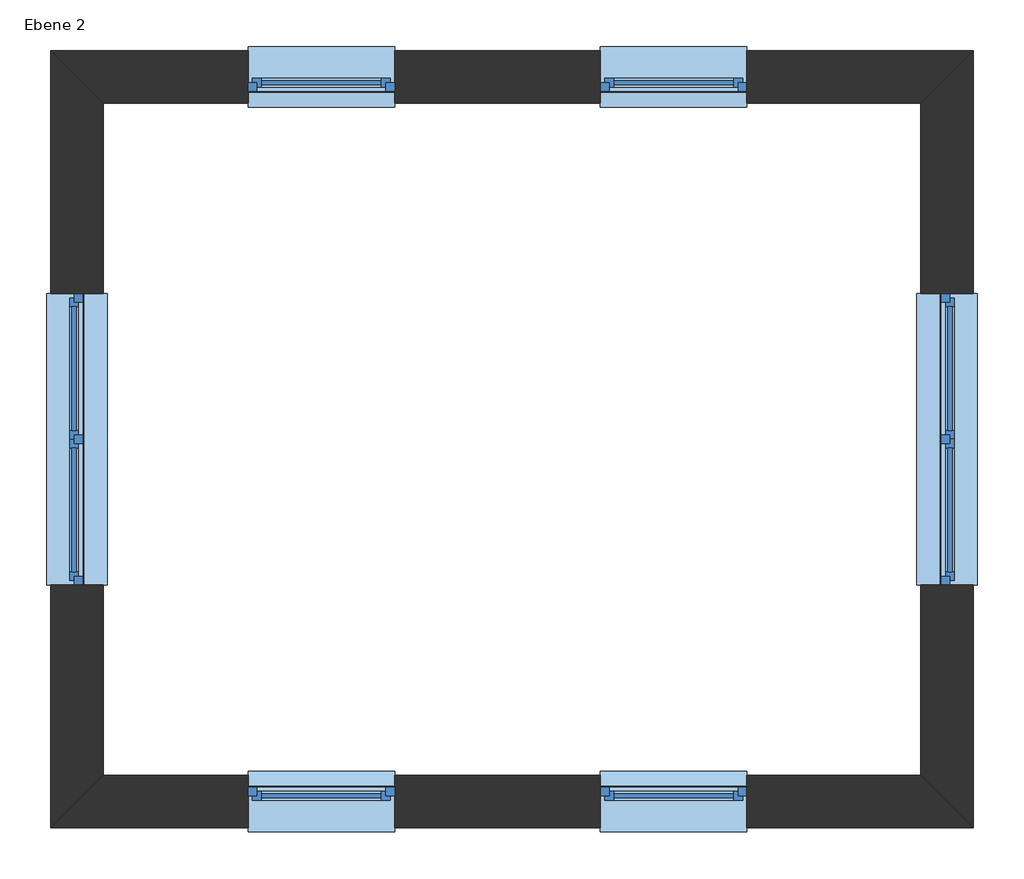
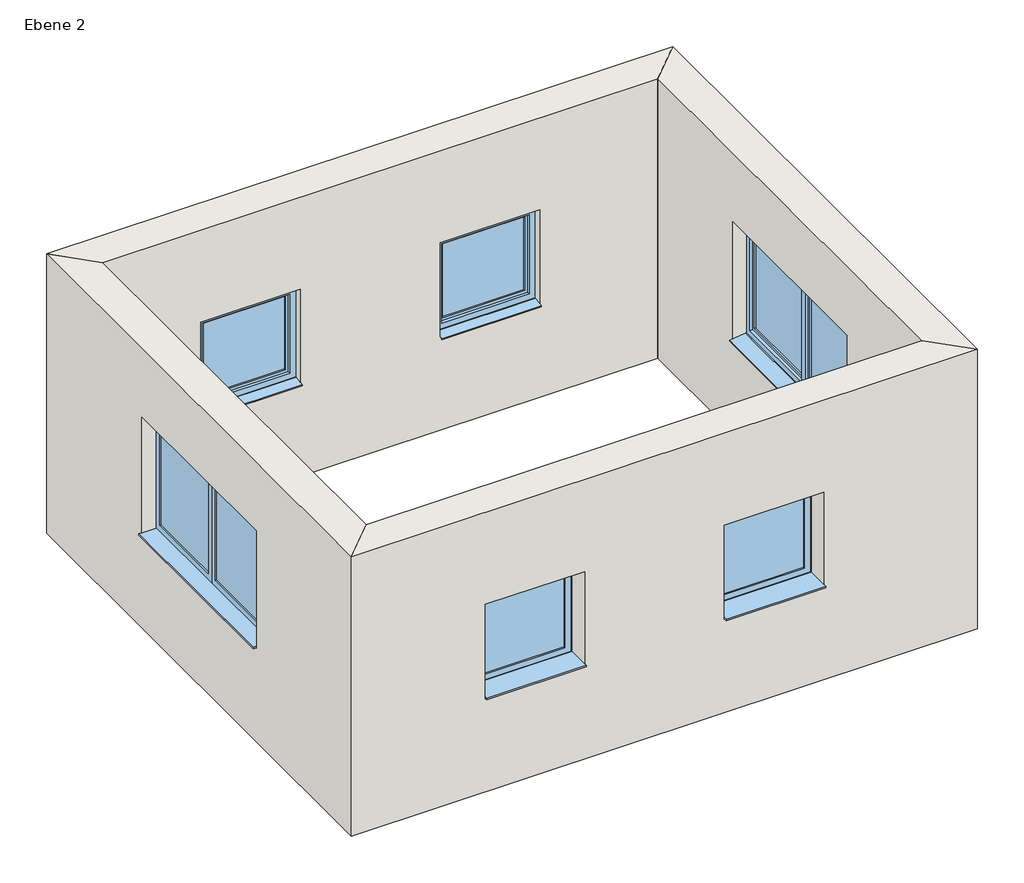
# One storey: 6 windows, 4 walls.
"""IFC4 building model written with IfcOpenShell, lengths in millimetres."""

import ifcopenshell
import ifcopenshell.guid

model = None  # the IFC model being written
_history = None  # IfcOwnerHistory: only IFC2X3 demands one
_inside = {}  # id of a spatial element -> (the spatial element, [elements in it])
_under = {}  # id of a project, library or spatial element -> (it, [spatial elements below it])
_declared = {}  # id of a project -> (the project, [libraries it declares])
_typed = {}  # id of a type object -> (the type object, [elements of that type])
_made_of = {}  # id of a material, layer set ... -> (it, [elements and type objects made of it])


def new_model(schema):
    """Start an empty IFC model of exactly this schema.

    Asked for "IFC4X3", IfcOpenShell would pick the latest addendum, in which some entities
    have other attributes; the version numbers below select the first issue.
    IFC2X3 requires an IfcOwnerHistory on every rooted entity: one is made here for all.
    """
    global model, _history
    if schema == "IFC4X3":
        model = ifcopenshell.file(schema_version=(4, 3, 0, 0))
    else:
        model = ifcopenshell.file(schema=schema)
    _inside.clear()
    _under.clear()
    _declared.clear()
    _typed.clear()
    _made_of.clear()
    _history = None
    if model.schema == "IFC2X3":
        org = make("IfcOrganization", Name="unknown")
        user = make(
            "IfcPersonAndOrganization",
            ThePerson=make("IfcPerson", FamilyName="unknown"),
            TheOrganization=org,
        )
        app = make(
            "IfcApplication",
            ApplicationDeveloper=org,
            Version="unknown",
            ApplicationFullName="unknown",
            ApplicationIdentifier="unknown",
        )
        _history = make(
            "IfcOwnerHistory",
            OwningUser=user,
            OwningApplication=app,
            ChangeAction="ADDED",
            CreationDate=0,
        )
    return model


def make(cls, **values):
    """One entity of the class cls with the attributes given. An attribute that is None is left unset."""
    return model.create_entity(
        cls, **{name: value for name, value in values.items() if value is not None}
    )


def rooted(cls, **values):
    """An entity with a GlobalId (a new one), such as an element, a storey or a relation."""
    return make(cls, GlobalId=ifcopenshell.guid.new(), OwnerHistory=_history, **values)


def si_unit(unit_type, name, prefix=None):
    """IfcSIUnit, for example si_unit("LENGTHUNIT", "METRE", prefix="MILLI")."""
    return make("IfcSIUnit", UnitType=unit_type, Prefix=prefix, Name=name)


def assignment(units):
    """IfcUnitAssignment: the units of a project."""
    return None if units is None else make("IfcUnitAssignment", Units=units)


def point(xyz):
    """IfcCartesianPoint."""
    return None if xyz is None else make("IfcCartesianPoint", Coordinates=xyz)


def direction(xyz):
    """IfcDirection."""
    return None if xyz is None else make("IfcDirection", DirectionRatios=xyz)


def frame(location, z_axis=None, x_axis=None):
    """IfcAxis2Placement3D, a coordinate frame: its origin and axes. An axis left out is left unset."""
    return make(
        "IfcAxis2Placement3D",
        Location=point(location),
        Axis=direction(z_axis),
        RefDirection=direction(x_axis),
    )


def origin():
    """The frame at (0, 0, 0) with its axes left unset."""
    return frame((0.0, 0.0, 0.0))


def place(relative_to, where):
    """IfcLocalPlacement: puts the frame where relative to a parent placement (None: the world)."""
    return make(
        "IfcLocalPlacement", PlacementRelTo=relative_to, RelativePlacement=where
    )


def context(
    kind, dimensions, precision=None, world=None, true_north=None, identifier=None
):
    """IfcGeometricRepresentationContext, for example the 3D "Model" context."""
    return make(
        "IfcGeometricRepresentationContext",
        ContextIdentifier=identifier,
        ContextType=kind,
        CoordinateSpaceDimension=dimensions,
        Precision=precision,
        WorldCoordinateSystem=world,
        TrueNorth=true_north,
    )


def project(units=None, contexts=None):
    """IfcProject with its units and contexts."""
    return rooted(
        "IfcProject",
        Name="project",
        RepresentationContexts=contexts,
        UnitsInContext=assignment(units),
    )


def spatial(cls, under=None, at=None, **own):
    """A site, building, storey or space (cls), placed at a placement, below another one or the project."""
    s = rooted(cls, ObjectPlacement=at, **own)
    if under is not None:
        _under.setdefault(under.id(), (under, []))[1].append(s)
    return s


def polyline(points):
    """IfcPolyline through the points."""
    return make("IfcPolyline", Points=[point(p) for p in points])


def outline(outer, holes=None, kind="AREA"):
    """IfcArbitraryClosedProfileDef: a profile drawn as a closed curve; with holes, ...WithVoids."""
    if holes is None:
        return make("IfcArbitraryClosedProfileDef", ProfileType=kind, OuterCurve=outer)
    return make(
        "IfcArbitraryProfileDefWithVoids",
        ProfileType=kind,
        OuterCurve=outer,
        InnerCurves=holes,
    )


def extrude(swept, where, along, depth):
    """IfcExtrudedAreaSolid: the profile swept, set in the frame where, extruded along a direction by depth."""
    return make(
        "IfcExtrudedAreaSolid",
        SweptArea=swept,
        Position=where,
        ExtrudedDirection=direction(along),
        Depth=depth,
    )


def faces_of(points, faces, orient=None, outer=None):
    """IfcFace entities. A face is a list of loops; a loop is a list of indices into points, from 0.

    orient and outer hold one flag for each loop. By default every Orientation is true, the
    first loop of a face is its IfcFaceOuterBound and the others are IfcFaceBound.
    """
    made = []
    for i, loops in enumerate(faces):
        bounds = []
        for j, loop in enumerate(loops):
            is_outer = j == 0 if outer is None else outer[i][j]
            bounds.append(
                make(
                    "IfcFaceOuterBound" if is_outer else "IfcFaceBound",
                    Bound=make("IfcPolyLoop", Polygon=[points[k] for k in loop]),
                    Orientation=True if orient is None else orient[i][j],
                )
            )
        made.append(make("IfcFace", Bounds=bounds))
    return made


def faceted_brep(points, faces, orient=None, outer=None, voids=None):
    """IfcFacetedBrep: a solid bounded by flat faces; with voids (closed shells), ...WithVoids."""
    shared = [point(p) for p in points]
    hull = make("IfcClosedShell", CfsFaces=faces_of(shared, faces, orient, outer))
    if voids is None:
        return make("IfcFacetedBrep", Outer=hull)
    return make(
        "IfcFacetedBrepWithVoids",
        Outer=hull,
        Voids=[
            make(cls, CfsFaces=faces_of(shared, fs, o, b)) for cls, fs, o, b in voids
        ],
    )


def shape(context_of_items, identifier, shape_type, items):
    """IfcShapeRepresentation: the items that make up one representation, for example the "Body"."""
    return make(
        "IfcShapeRepresentation",
        ContextOfItems=context_of_items,
        RepresentationIdentifier=identifier,
        RepresentationType=shape_type,
        Items=items,
    )


def source(mapping_origin, context_of_items, identifier, shape_type, items):
    """IfcRepresentationMap: a shape defined once, which mapped items show again and again."""
    return make(
        "IfcRepresentationMap",
        MappingOrigin=mapping_origin,
        MappedRepresentation=shape(context_of_items, identifier, shape_type, items),
    )


def transform(
    local_origin,
    x_axis=None,
    y_axis=None,
    z_axis=None,
    scale=None,
    scale2=None,
    scale3=None,
    uniform=True,
):
    """IfcCartesianTransformationOperator3D, or its non-uniform kind. x_axis, y_axis, z_axis: its Axis1, 2, 3."""
    if uniform:
        return make(
            "IfcCartesianTransformationOperator3D",
            Axis1=direction(x_axis),
            Axis2=direction(y_axis),
            LocalOrigin=point(local_origin),
            Scale=scale,
            Axis3=direction(z_axis),
        )
    return make(
        "IfcCartesianTransformationOperator3DnonUniform",
        Axis1=direction(x_axis),
        Axis2=direction(y_axis),
        LocalOrigin=point(local_origin),
        Scale=scale,
        Axis3=direction(z_axis),
        Scale2=scale2,
        Scale3=scale3,
    )


def mapped(mapping_source, mapping_target):
    """IfcMappedItem: shows the shape of a source again, moved by a transform."""
    return make(
        "IfcMappedItem", MappingSource=mapping_source, MappingTarget=mapping_target
    )


def made_of(thing, what):
    """Note that an element or type object is made of a material, layer set ...; save() writes the relation."""
    if what is not None:
        _made_of.setdefault(what.id(), (what, []))[1].append(thing)
    return thing


def element(
    cls,
    number,
    at=None,
    inside=None,
    cuts=None,
    type_object=None,
    material=None,
    context=None,
    identifier="Body",
    shape_type=None,
    held_by="IfcProductDefinitionShape",
    body=None,
    shapes=None,
    **own,
):
    """One element of the class cls, such as IfcWall. Its Tag is "e" and its number.

    at: its placement. inside: the storey or other place that contains it. cuts: it is an
    opening in that element (IfcRelVoidsElement). A single representation is given by context,
    identifier, shape_type and body (its items); several are given by shapes. held_by: the class
    of the entity that holds the representations. save() writes the other relations.
    """
    e = rooted(cls, Tag="e%d" % number, ObjectPlacement=at, **own)
    if body is not None:
        shapes = [shape(context, identifier, shape_type, body)]
    if shapes is not None:
        e.Representation = make(held_by, Representations=shapes)
    if inside is not None:
        _inside.setdefault(inside.id(), (inside, []))[1].append(e)
    if cuts is not None:
        rooted(
            "IfcRelVoidsElement", RelatingBuildingElement=cuts, RelatedOpeningElement=e
        )
    if type_object is not None:
        _typed.setdefault(type_object.id(), (type_object, []))[1].append(e)
    return made_of(e, material)


def aggregate(whole, parts):
    """IfcRelAggregates: a whole, such as a stair, and the parts it consists of."""
    return rooted("IfcRelAggregates", RelatingObject=whole, RelatedObjects=parts)


def save(model, path):
    """Write the relations noted so far, then the file.

    IfcRelAggregates (storeys below a building ...), IfcRelContainedInSpatialStructure (elements
    in a storey), IfcRelDefinesByType, IfcRelAssociatesMaterial and IfcRelDeclares: one each for
    every whole, place, type object, material and project.
    """
    for whole, parts in _under.values():
        aggregate(whole, parts)
    for where, things in _inside.values():
        rooted(
            "IfcRelContainedInSpatialStructure",
            RelatedElements=things,
            RelatingStructure=where,
        )
    for kind, things in _typed.values():
        rooted("IfcRelDefinesByType", RelatedObjects=things, RelatingType=kind)
    for what, things in _made_of.values():
        rooted("IfcRelAssociatesMaterial", RelatedObjects=things, RelatingMaterial=what)
    for by, libraries in _declared.values():
        rooted("IfcRelDeclares", RelatingContext=by, RelatedDefinitions=libraries)
    model.write(path)


def fenster_1_flg_variabel_fenster_1_flg_variabel_3_8a378bad(model_context):
    return source(origin(), model_context, "Body", "SolidModel", [
        extrude(outline(polyline([(2010.0, 505.0), (2010.0, -505.0), (1000.0, -505.0), (1000.0, 505.0), (2010.0, 505.0)]), holes=[polyline([(1930.0, 445.0), (1080.0, 445.0), (1080.0, -445.0), (1930.0, -445.0), (1930.0, 445.0)])]), frame((0.0, 40.0, 0.0), z_axis=(0.0, 1.0, 0.0), x_axis=(0.0, 0.0, 1.0)), (0.0, 0.0, 1.0), 60.0),
        faceted_brep([(475.0, 40.0, 1960.0), (475.0, 10.0, 1960.0), (475.0, 10.0, 1050.0), (475.0, 40.0, 1050.0), (-475.0, 10.0, 1960.0), (-475.0, 10.0, 1050.0), (415.0, 10.0, 1110.0), (-415.0, 10.0, 1110.0), (-415.0, 10.0, 1900.0), (415.0, 10.0, 1900.0), (-475.0, 40.0, 1050.0), (-475.0, 40.0, 1960.0), (445.0, 40.0, 1930.0), (-445.0, 40.0, 1930.0), (-445.0, 40.0, 1080.0), (445.0, 40.0, 1080.0), (445.0, 70.0, 1930.0), (445.0, 70.0, 1080.0), (-445.0, 70.0, 1080.0), (-445.0, 70.0, 1930.0), (415.0, 70.0, 1900.0), (-415.0, 70.0, 1900.0), (-415.0, 70.0, 1110.0), (415.0, 70.0, 1110.0)], [[[0, 1, 2, 3]], [[1, 4, 5, 2], [6, 7, 8, 9]], [[3, 2, 5, 10]], [[3, 10, 11, 0], [12, 13, 14, 15]], [[16, 12, 15, 17]], [[17, 15, 14, 18]], [[17, 18, 19, 16], [20, 21, 22, 23]], [[9, 20, 23, 6]], [[6, 23, 22, 7]], [[10, 5, 4, 11]], [[18, 14, 13, 19]], [[7, 22, 21, 8]], [[11, 4, 1, 0]], [[19, 13, 12, 16]], [[8, 21, 20, 9]]]),
        extrude(outline(polyline([(-505.0, -210.0), (-505.0, 40.0), (505.0, 40.0), (505.0, -210.0), (-505.0, -210.0)])), frame((0.0, 0.0, 1005.0), z_axis=(0.0, 0.0, 1.0), x_axis=(1.0, 0.0, 0.0)), (0.0, 0.0, 1.0), 15.0),
        extrude(outline(polyline([(110.0221543, 1020.0), (210.0, 1000.0), (210.0, 990.0), (208.0, 990.0), (208.0, 998.3604634), (109.8240723, 1018.0), (100.0, 1018.0), (100.0, 1020.0), (110.0221543, 1020.0)])), frame((-505.0, 0.0, 0.0), z_axis=(1.0, 0.0, 0.0), x_axis=(0.0, 1.0, 0.0)), (0.0, 0.0, 1.0), 1010.0),
        extrude(outline(polyline([(415.0, 25.0), (-415.0, 25.0), (-415.0, 55.0), (415.0, 55.0), (415.0, 25.0)])), frame((0.0, 0.0, 1110.0), z_axis=(0.0, 0.0, 1.0), x_axis=(1.0, 0.0, 0.0)), (0.0, 0.0, 1.0), 790.0),
    ])


def fenster_2_flg_variabel_fenster_2_flg_variabel_3_03287464(model_context):
    return source(origin(), model_context, "Body", "SolidModel", [
        extrude(outline(polyline([(60.0, -5.0), (915.0, -5.0), (915.0, -35.0), (60.0, -35.0), (60.0, -5.0)])), frame((0.0, 0.0, 1110.0), z_axis=(0.0, 0.0, 1.0), x_axis=(1.0, 0.0, 0.0)), (0.0, 0.0, 1.0), 1040.0),
        extrude(outline(polyline([(-915.0, -5.0), (-60.0, -5.0), (-60.0, -35.0), (-915.0, -35.0), (-915.0, -5.0)])), frame((0.0, 0.0, 1110.0), z_axis=(0.0, 0.0, 1.0), x_axis=(1.0, 0.0, 0.0)), (0.0, 0.0, 1.0), 1040.0),
        extrude(outline(polyline([(-1005.0, -210.0), (-1005.0, -20.0), (1005.0, -20.0), (1005.0, -210.0), (-1005.0, -210.0)])), frame((0.0, 0.0, 1005.0), z_axis=(0.0, 0.0, 1.0), x_axis=(1.0, 0.0, 0.0)), (0.0, 0.0, 1.0), 15.0),
        extrude(outline(polyline([(50.0221543, 1020.0), (210.0, 1000.0), (210.0, 990.0), (208.0, 990.0), (208.0, 998.3604634), (49.8240723, 1018.0), (40.0, 1018.0), (40.0, 1020.0), (50.0221543, 1020.0)])), frame((-1005.0, 0.0, 0.0), z_axis=(1.0, 0.0, 0.0), x_axis=(0.0, 1.0, 0.0)), (0.0, 0.0, 1.0), 2010.0),
        extrude(outline(polyline([(30.0, -20.0), (-30.0, -20.0), (-30.0, 40.0), (30.0, 40.0), (30.0, -20.0)])), frame((0.0, 0.0, 1080.0), z_axis=(0.0, 0.0, 1.0), x_axis=(1.0, 0.0, 0.0)), (0.0, 0.0, 1.0), 1100.0),
        extrude(outline(polyline([(2260.0, -1005.0), (1000.0, -1005.0), (1000.0, 1005.0), (2260.0, 1005.0), (2260.0, -1005.0)]), holes=[polyline([(2180.0, -945.0), (2180.0, 945.0), (1080.0, 945.0), (1080.0, -945.0), (2180.0, -945.0)])]), frame((0.0, -20.0, 0.0), z_axis=(0.0, 1.0, 0.0), x_axis=(0.0, 0.0, 1.0)), (0.0, 0.0, 1.0), 60.0),
        faceted_brep([(-945.0, -20.0, 1080.0), (-945.0, 10.0, 1080.0), (-30.0, 10.0, 1080.0), (-30.0, -20.0, 1080.0), (-30.0, 10.0, 2180.0), (-30.0, -20.0, 2180.0), (-945.0, 10.0, 2180.0), (-60.0, 10.0, 2150.0), (-915.0, 10.0, 2150.0), (-915.0, 10.0, 1110.0), (-60.0, 10.0, 1110.0), (0.0, -20.0, 1050.0), (-975.0, -20.0, 1050.0), (-975.0, -20.0, 2210.0), (0.0, -20.0, 2210.0), (-945.0, -20.0, 2180.0), (-975.0, -50.0, 1050.0), (0.0, -50.0, 1050.0), (0.0, -50.0, 2210.0), (-975.0, -50.0, 2210.0), (-60.0, -50.0, 1110.0), (-915.0, -50.0, 1110.0), (-915.0, -50.0, 2150.0), (-60.0, -50.0, 2150.0)], [[[0, 1, 2, 3]], [[3, 2, 4, 5]], [[2, 1, 6, 4], [7, 8, 9, 10]], [[11, 12, 13, 14], [5, 15, 0, 3]], [[16, 12, 11, 17]], [[17, 11, 14, 18]], [[18, 19, 16, 17], [20, 21, 22, 23]], [[9, 21, 20, 10]], [[10, 20, 23, 7]], [[15, 6, 1, 0]], [[19, 13, 12, 16]], [[8, 22, 21, 9]], [[5, 4, 6, 15]], [[18, 14, 13, 19]], [[7, 23, 22, 8]]]),
        faceted_brep([(30.0, -20.0, 1080.0), (30.0, 10.0, 1080.0), (945.0, 10.0, 1080.0), (945.0, -20.0, 1080.0), (945.0, 10.0, 2180.0), (945.0, -20.0, 2180.0), (30.0, 10.0, 2180.0), (915.0, 10.0, 2150.0), (60.0, 10.0, 2150.0), (60.0, 10.0, 1110.0), (915.0, 10.0, 1110.0), (975.0, -20.0, 1050.0), (0.0, -20.0, 1050.0), (0.0, -20.0, 2210.0), (975.0, -20.0, 2210.0), (30.0, -20.0, 2180.0), (0.0, -50.0, 1050.0), (975.0, -50.0, 1050.0), (975.0, -50.0, 2210.0), (0.0, -50.0, 2210.0), (915.0, -50.0, 1110.0), (60.0, -50.0, 1110.0), (60.0, -50.0, 2150.0), (915.0, -50.0, 2150.0)], [[[0, 1, 2, 3]], [[3, 2, 4, 5]], [[2, 1, 6, 4], [7, 8, 9, 10]], [[11, 12, 13, 14], [5, 15, 0, 3]], [[16, 12, 11, 17]], [[17, 11, 14, 18]], [[18, 19, 16, 17], [20, 21, 22, 23]], [[9, 21, 20, 10]], [[10, 20, 23, 7]], [[15, 6, 1, 0]], [[19, 13, 12, 16]], [[8, 22, 21, 9]], [[5, 4, 6, 15]], [[18, 14, 13, 19]], [[7, 23, 22, 8]]]),
    ])


model = new_model("IFC4")

# Units and contexts
model_context = context("Model", 3, world=origin())
ifc_project = project(units=[si_unit("LENGTHUNIT", "METRE", prefix="MILLI")], contexts=[model_context])

# Site, building, storey
site = spatial("IfcSite", under=ifc_project)
building = spatial("IfcBuilding", under=site)
storey = spatial("IfcBuildingStorey", under=building, Name="Ebene 2", Elevation=6000.0)

# Walls
placement = place(None, origin())
element("IfcWall", 1, ObjectType="MW 24.0 WD 12.0", at=placement, inside=storey, context=model_context, shape_type="Brep", body=[
    faceted_brep([(-3766.4979049, 4044.3692517, 6000.0), (1873.5020951, 4044.3692517, 6000.0), (1873.5020951, 4044.3692517, 9000.0), (-3766.4979049, 4044.3692517, 9000.0), (673.5020951, 4044.3692517, 7000.0), (-336.4979049, 4044.3692517, 7000.0), (-336.4979049, 4044.3692517, 8010.0), (673.5020951, 4044.3692517, 8010.0), (-1756.4979049, 4044.3692517, 7000.0), (-2766.4979049, 4044.3692517, 7000.0), (-2766.4979049, 4044.3692517, 8010.0), (-1756.4979049, 4044.3692517, 8010.0), (-4126.4979049, 4404.3692517, 6000.0), (-4126.4979049, 4404.3692517, 9000.0), (2233.5020951, 4404.3692517, 9000.0), (2233.5020951, 4404.3692517, 6000.0), (673.5020951, 4404.3692517, 7000.0), (673.5020951, 4404.3692517, 8010.0), (-336.4979049, 4404.3692517, 8010.0), (-336.4979049, 4404.3692517, 7000.0), (-1756.4979049, 4404.3692517, 7000.0), (-1756.4979049, 4404.3692517, 8010.0), (-2766.4979049, 4404.3692517, 8010.0), (-2766.4979049, 4404.3692517, 7000.0)], [[[0, 1, 2, 3], [4, 5, 6, 7], [8, 9, 10, 11]], [[12, 13, 14, 15], [16, 17, 18, 19], [20, 21, 22, 23]], [[1, 0, 12, 15]], [[3, 2, 14, 13]], [[2, 1, 15, 14]], [[0, 3, 13, 12]], [[17, 16, 4, 7]], [[18, 17, 7, 6]], [[19, 18, 6, 5]], [[16, 19, 5, 4]], [[21, 20, 8, 11]], [[22, 21, 11, 10]], [[23, 22, 10, 9]], [[20, 23, 9, 8]]]),
])
element("IfcWall", 2, ObjectType="MW 24.0 WD 12.0", at=placement, inside=storey, context=model_context, shape_type="Brep", body=[
    faceted_brep([(1873.5020951, 4044.3692517, 6000.0), (1873.5020951, -595.6307483, 6000.0), (1873.5020951, -595.6307483, 9000.0), (1873.5020951, 4044.3692517, 9000.0), (1873.5020951, 719.3692517, 7000.0), (1873.5020951, 2729.3692517, 7000.0), (1873.5020951, 2729.3692517, 8260.0), (1873.5020951, 719.3692517, 8260.0), (2233.5020951, 4404.3692517, 6000.0), (2233.5020951, 4404.3692517, 9000.0), (2233.5020951, -955.6307483, 9000.0), (2233.5020951, -955.6307483, 6000.0), (2233.5020951, 719.3692517, 7000.0), (2233.5020951, 719.3692517, 8260.0), (2233.5020951, 2729.3692517, 8260.0), (2233.5020951, 2729.3692517, 7000.0)], [[[0, 1, 2, 3], [4, 5, 6, 7]], [[8, 9, 10, 11], [12, 13, 14, 15]], [[1, 0, 8, 11]], [[3, 2, 10, 9]], [[0, 3, 9, 8]], [[2, 1, 11, 10]], [[13, 12, 4, 7]], [[14, 13, 7, 6]], [[15, 14, 6, 5]], [[12, 15, 5, 4]]]),
])
element("IfcWall", 3, ObjectType="MW 24.0 WD 12.0", at=placement, inside=storey, context=model_context, shape_type="Brep", body=[
    faceted_brep([(1873.5020951, -595.6307483, 6000.0), (-3766.4979049, -595.6307483, 6000.0), (-3766.4979049, -595.6307483, 9000.0), (1873.5020951, -595.6307483, 9000.0), (-336.4979049, -595.6307483, 7000.0), (673.5020951, -595.6307483, 7000.0), (673.5020951, -595.6307483, 8010.0), (-336.4979049, -595.6307483, 8010.0), (-2766.4979049, -595.6307483, 7000.0), (-1756.4979049, -595.6307483, 7000.0), (-1756.4979049, -595.6307483, 8010.0), (-2766.4979049, -595.6307483, 8010.0), (2233.5020951, -955.6307483, 6000.0), (2233.5020951, -955.6307483, 9000.0), (-4126.4979049, -955.6307483, 9000.0), (-4126.4979049, -955.6307483, 6000.0), (-336.4979049, -955.6307483, 7000.0), (-336.4979049, -955.6307483, 8010.0), (673.5020951, -955.6307483, 8010.0), (673.5020951, -955.6307483, 7000.0), (-2766.4979049, -955.6307483, 7000.0), (-2766.4979049, -955.6307483, 8010.0), (-1756.4979049, -955.6307483, 8010.0), (-1756.4979049, -955.6307483, 7000.0)], [[[0, 1, 2, 3], [4, 5, 6, 7], [8, 9, 10, 11]], [[12, 13, 14, 15], [16, 17, 18, 19], [20, 21, 22, 23]], [[1, 0, 12, 15]], [[3, 2, 14, 13]], [[0, 3, 13, 12]], [[2, 1, 15, 14]], [[17, 16, 4, 7]], [[18, 17, 7, 6]], [[19, 18, 6, 5]], [[16, 19, 5, 4]], [[21, 20, 8, 11]], [[22, 21, 11, 10]], [[23, 22, 10, 9]], [[20, 23, 9, 8]]]),
])
element("IfcWall", 4, ObjectType="MW 24.0 WD 12.0", at=placement, inside=storey, context=model_context, shape_type="Brep", body=[
    faceted_brep([(-3766.4979049, -595.6307483, 6000.0), (-3766.4979049, 4044.3692517, 6000.0), (-3766.4979049, 4044.3692517, 9000.0), (-3766.4979049, -595.6307483, 9000.0), (-3766.4979049, 2729.3692517, 7000.0), (-3766.4979049, 719.3692517, 7000.0), (-3766.4979049, 719.3692517, 8260.0), (-3766.4979049, 2729.3692517, 8260.0), (-4126.4979049, -955.6307483, 6000.0), (-4126.4979049, -955.6307483, 9000.0), (-4126.4979049, 4404.3692517, 9000.0), (-4126.4979049, 4404.3692517, 6000.0), (-4126.4979049, 2729.3692517, 7000.0), (-4126.4979049, 2729.3692517, 8260.0), (-4126.4979049, 719.3692517, 8260.0), (-4126.4979049, 719.3692517, 7000.0)], [[[0, 1, 2, 3], [4, 5, 6, 7]], [[8, 9, 10, 11], [12, 13, 14, 15]], [[1, 0, 8, 11]], [[3, 2, 10, 9]], [[2, 1, 11, 10]], [[0, 3, 9, 8]], [[13, 12, 4, 7]], [[14, 13, 7, 6]], [[15, 14, 6, 5]], [[12, 15, 5, 4]]]),
])

# Windows
fenster_1_flg_variabel_fenster_1_flg_variabel_3_shape = fenster_1_flg_variabel_fenster_1_flg_variabel_3_8a378bad(model_context)
element("IfcWindow", 5, ObjectType="Fenster 1-flg - Variabel : Fenster 1-flg - Variabel 3", at=placement, inside=storey, context=model_context, shape_type="MappedRepresentation", body=[
    mapped(fenster_1_flg_variabel_fenster_1_flg_variabel_3_shape, transform((168.5020951, -775.6307483, 6000.0), x_axis=(1.0, 0.0, 0.0), y_axis=(0.0, 1.0, 0.0), z_axis=(0.0, 0.0, 1.0))),
])
element("IfcWindow", 6, ObjectType="Fenster 1-flg - Variabel : Fenster 1-flg - Variabel 3", at=placement, inside=storey, context=model_context, shape_type="MappedRepresentation", body=[
    mapped(fenster_1_flg_variabel_fenster_1_flg_variabel_3_shape, transform((-2261.4979049, -775.6307483, 6000.0), x_axis=(1.0, 0.0, 0.0), y_axis=(0.0, 1.0, 0.0), z_axis=(0.0, 0.0, 1.0))),
])
element("IfcWindow", 7, ObjectType="Fenster 1-flg - Variabel : Fenster 1-flg - Variabel 3", at=placement, inside=storey, context=model_context, shape_type="MappedRepresentation", body=[
    mapped(fenster_1_flg_variabel_fenster_1_flg_variabel_3_shape, transform((168.5020951, 4224.3692517, 6000.0), x_axis=(-1.0, 0.0, 0.0), y_axis=(0.0, -1.0, 0.0), z_axis=(0.0, 0.0, 1.0))),
])
element("IfcWindow", 8, ObjectType="Fenster 1-flg - Variabel : Fenster 1-flg - Variabel 3", at=placement, inside=storey, context=model_context, shape_type="MappedRepresentation", body=[
    mapped(fenster_1_flg_variabel_fenster_1_flg_variabel_3_shape, transform((-2261.4979049, 4224.3692517, 6000.0), x_axis=(-1.0, 0.0, 0.0), y_axis=(0.0, -1.0, 0.0), z_axis=(0.0, 0.0, 1.0))),
])
fenster_2_flg_variabel_fenster_2_flg_variabel_3_shape = fenster_2_flg_variabel_fenster_2_flg_variabel_3_03287464(model_context)
element("IfcWindow", 9, ObjectType="Fenster 2-flg - Variabel : Fenster 2-flg - Variabel 3", at=placement, inside=storey, context=model_context, shape_type="MappedRepresentation", body=[
    mapped(fenster_2_flg_variabel_fenster_2_flg_variabel_3_shape, transform((2053.5020951, 1724.3692517, 6000.0), x_axis=(0.0, 1.0, 0.0), y_axis=(-1.0, 0.0, 0.0), z_axis=(0.0, 0.0, 1.0))),
])
element("IfcWindow", 10, ObjectType="Fenster 2-flg - Variabel : Fenster 2-flg - Variabel 3", at=placement, inside=storey, context=model_context, shape_type="MappedRepresentation", body=[
    mapped(fenster_2_flg_variabel_fenster_2_flg_variabel_3_shape, transform((-3946.4979049, 1724.3692517, 6000.0), x_axis=(0.0, -1.0, 0.0), y_axis=(1.0, 0.0, 0.0), z_axis=(0.0, 0.0, 1.0))),
])

save(model, "model.ifc")

# Revit data of these elements
# Type "MW 24.0 WD 12.0"
#   Type Comments = "Mehrschaliges Mauerwerk"
#   Description = "Mauerwerk 24.0 cm, Wärmedämmung 12.0 cm"
#   Layers, outside or top first: 0.120 m "Wärmedämmung - hart" (function 3); 0.240 m "Mauerwerk - Ziegel, verputzt" (function 1)
# Type "Fenster 1-flg - Variabel : Fenster 1-flg - Variabel 3"
#   Type Mark = "52"
#   Operation = "SinglePanel"
#   Construction Type Id = "GSP4R"
#   Keynote = "16.05.01"
#   Analytic Construction = "1/8 Zoll Pilkington-Verglasung einfach"
#   Cost = 78.2
#   Visual Light Transmittance = 0.9
#   Höhe oberer  Rahmen = 0.080 m
#   Solar Heat Gain Coefficient = 0.86
#   Tiefe Flügel = 0.060 m
#   Rough Width [instance default] = 1.010 m
#   Rough Height [instance default] = 1.010 m
#   Rahmenhöhe unten = 0.080 m
#   Heat Transfer Coefficient (U) = 6.7069 W/(m²·K)
#   Rahmentiefe = 0.060 m
#   Rahmenbreite = 0.060 m
#   Height [instance default] = 1.010 m
#   Flügelbreite = 0.060 m
#   Einbautiefe (von außen) [instance default] = 0.080 m
#   Width [instance default] = 1.010 m
#   Define Thermal Properties by = 1
#   Öffnungsrichtung oben [instance default] = yes
#   Öffnungsrichtung in Draufsicht anzeigen [instance default] = no
#   Klappflügel [instance default] = no
#   Drehflügel 1 [instance default] = yes
#   Fensterflügel [instance default] = none
#   Innere Fensterbank [instance default] = none
#   Glas [instance default] = none
#   Bild [instance default] = none
#   Äußere Fensterbank [instance default] = none
#   Wall Closure = (empty or 0)
# Type "Fenster 2-flg - Variabel : Fenster 2-flg - Variabel 3"
#   Type Mark = "53"
#   Operation = "DoublePanelVertical"
#   Construction Type Id = "GSP4R"
#   Keynote = "16.05.01"
#   Analytic Construction = "1/8 Zoll Pilkington-Verglasung einfach"
#   Cost = 130.98
#   Visual Light Transmittance = 0.9
#   Solar Heat Gain Coefficient = 0.78
#   Rough Width [instance default] = 2.010 m
#   Rough Height [instance default] = 1.260 m
#   Heat Transfer Coefficient (U) = 3.6886 W/(m²·K)
#   Rahmentiefe = 0.060 m
#   Rahmenhöhe unten = 0.080 m
#   Höhe oberer  Rahmen = 0.080 m
#   Rahmenbreite = 0.060 m
#   Height [instance default] = 1.260 m
#   Tiefe Flügel = 0.060 m
#   Flügelbreite = 0.060 m
#   Einbautiefe (von außen) [instance default] = 0.140 m
#   Width [instance default] = 2.010 m
#   Define Thermal Properties by = 1
#   Öffnungsrichtung oben [instance default] = yes
#   Öffnungsrichtung in Draufsicht anzeigen [instance default] = no
#   Drehflügel 1 [instance default] = yes
#   Bild [instance default] = none
#   Glas [instance default] = none
#   Fensterflügel [instance default] = none
#   Äußere Fensterbank [instance default] = none
#   Innere Fensterbank [instance default] = none
#   Wall Closure = (empty or 0)
# Elements 1, 2, 3, 4 (IfcWall, "MW 24.0 WD 12.0")
#   Comments = ""
#   Top Offset = 0.000 m
#   Base Offset = 0.000 m
#   Unconnected Height = 3.000 m
#   wall height = 3.000 m
#   Phase Created = Phase 1
#   Base Constraint = Ebene 2
#   Materials on its faces: "Vorgabe - Wand", "Mauerwerk - Ziegel, verputzt", "Wärmedämmung - hart"
# Element 5 (IfcWindow, "Fenster 1-flg - Variabel : Fenster 1-flg - Variabel 3")
#   Mark = "10"
#   Rough Height = 1.010 m
#   Rough Width = 1.010 m
#   Height = 1.010 m
#   Einbautiefe (von außen) = 0.080 m
#   Width = 1.010 m
#   Öffnungsrichtung oben = yes
#   Öffnungsrichtung in Draufsicht anzeigen = no
#   Klappflügel = no
#   Drehflügel 1 = yes
#   Äußere Fensterbank = none
#   Innere Fensterbank = none
#   Glas = none
#   Fensterflügel = none
#   Bild = none
#   Phase Created = Phase 1
#   Materials on its faces: "Kunststoff - Weiß", "Holz - Birke", "Glas"
# Element 6 (IfcWindow, "Fenster 1-flg - Variabel : Fenster 1-flg - Variabel 3")
#   Mark = "11"
#   Rough Height = 1.010 m
#   Rough Width = 1.010 m
#   Height = 1.010 m
#   Einbautiefe (von außen) = 0.080 m
#   Width = 1.010 m
#   Öffnungsrichtung oben = yes
#   Öffnungsrichtung in Draufsicht anzeigen = no
#   Klappflügel = no
#   Drehflügel 1 = yes
#   Äußere Fensterbank = none
#   Innere Fensterbank = none
#   Glas = none
#   Fensterflügel = none
#   Bild = none
#   Phase Created = Phase 1
#   Materials on its faces: "Kunststoff - Weiß", "Holz - Birke", "Glas"
# Element 7 (IfcWindow, "Fenster 1-flg - Variabel : Fenster 1-flg - Variabel 3")
#   Mark = "12"
#   Rough Height = 1.010 m
#   Rough Width = 1.010 m
#   Height = 1.010 m
#   Einbautiefe (von außen) = 0.080 m
#   Width = 1.010 m
#   Öffnungsrichtung oben = yes
#   Öffnungsrichtung in Draufsicht anzeigen = no
#   Klappflügel = no
#   Drehflügel 1 = yes
#   Äußere Fensterbank = none
#   Innere Fensterbank = none
#   Glas = none
#   Fensterflügel = none
#   Bild = none
#   Phase Created = Phase 1
#   Materials on its faces: "Kunststoff - Weiß", "Holz - Birke", "Glas"
# Element 8 (IfcWindow, "Fenster 1-flg - Variabel : Fenster 1-flg - Variabel 3")
#   Mark = "13"
#   Rough Height = 1.010 m
#   Rough Width = 1.010 m
#   Height = 1.010 m
#   Einbautiefe (von außen) = 0.080 m
#   Width = 1.010 m
#   Öffnungsrichtung oben = yes
#   Öffnungsrichtung in Draufsicht anzeigen = no
#   Klappflügel = no
#   Drehflügel 1 = yes
#   Äußere Fensterbank = none
#   Innere Fensterbank = none
#   Glas = none
#   Fensterflügel = none
#   Bild = none
#   Phase Created = Phase 1
#   Materials on its faces: "Kunststoff - Weiß", "Holz - Birke", "Glas"
# Element 9 (IfcWindow, "Fenster 2-flg - Variabel : Fenster 2-flg - Variabel 3")
#   Mark = "14"
#   Rough Height = 1.260 m
#   Rough Width = 2.010 m
#   Height = 1.260 m
#   Einbautiefe (von außen) = 0.140 m
#   Width = 2.010 m
#   Öffnungsrichtung oben = yes
#   Öffnungsrichtung in Draufsicht anzeigen = no
#   Drehflügel 1 = yes
#   Äußere Fensterbank = none
#   Innere Fensterbank = none
#   Glas = none
#   Fensterflügel = none
#   Bild = none
#   Phase Created = Phase 1
#   Materials on its faces: "Kunststoff - Weiß", "Glas", "Holz - Birke"
# Element 10 (IfcWindow, "Fenster 2-flg - Variabel : Fenster 2-flg - Variabel 3")
#   Mark = "15"
#   Rough Height = 1.260 m
#   Rough Width = 2.010 m
#   Height = 1.260 m
#   Einbautiefe (von außen) = 0.140 m
#   Width = 2.010 m
#   Öffnungsrichtung oben = yes
#   Öffnungsrichtung in Draufsicht anzeigen = no
#   Drehflügel 1 = yes
#   Äußere Fensterbank = none
#   Innere Fensterbank = none
#   Glas = none
#   Fensterflügel = none
#   Bild = none
#   Phase Created = Phase 1
#   Materials on its faces: "Kunststoff - Weiß", "Glas", "Holz - Birke"
# Materials
#   "Wärmedämmung - hart": class "Stuck", colour RGB 255 255 255, transparency 0, Description = "Äußere Oberfläche", Cost = 0
#   "Mauerwerk - Ziegel, verputzt": class "Stuck", colour RGB 247 247 247, transparency 0, Cost = 0
#   "Vorgabe - Wand": class "Stuck", colour RGB 128 128 128, transparency 0, Description = "Äußere Oberfläche", Cost = 0
#   "Kunststoff - Weiß": class "Kunststoff", colour RGB 249 249 249, transparency 0, Cost = 0
#   "Holz - Birke": class "Holz", colour RGB 213 164 103, transparency 0, Cost = 0
#   "Glas": class "Glas", colour RGB 0 0 255, transparency 0.75, Comments = "Render-Darstellung nicht aktualisiert ", Cost = 0
